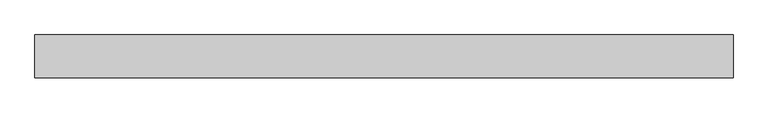
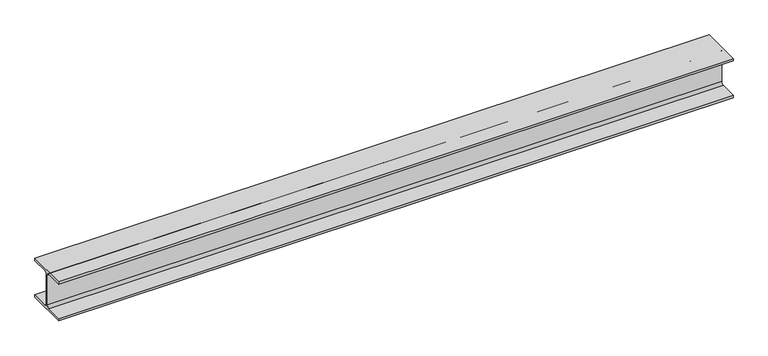
"""IFC4 building model written with IfcOpenShell, lengths in millimetres: beam geometry, 0912_Steel Framing_H-KSD3502 : H_SB_ASB_H-200x200x8x12."""

from ifc_helpers import new_model, si_unit, point, frame, frame_2d, origin, place, context, project, spatial, polyline, circle_curve, trimmed, segment, composite_curve, outline, extrude, source, transform, mapped, element, save


def beam_1c4525a5(model_context):
    return source(origin(), model_context, "Body", "SweptSolid", [
        extrude(outline(composite_curve([segment(polyline([(100.0, -88.0), (100.0, -100.0), (-100.0, -100.0), (-100.0, -88.0), (-17.0, -88.0)]), True, "CONTINUOUS"), segment(trimmed(circle_curve(frame_2d((-17.0, -75.0)), 13.0), [point((-17.0, -88.0))], [point((-4.0, -75.0))], True, "CARTESIAN"), True, "CONTINUOUS"), segment(polyline([(-4.0, -75.0), (-4.0, 75.0)]), True, "CONTINUOUS"), segment(trimmed(circle_curve(frame_2d((-17.0, 75.0)), 13.0), [point((-4.0, 75.0))], [point((-17.0, 88.0))], True, "CARTESIAN"), True, "CONTINUOUS"), segment(polyline([(-17.0, 88.0), (-100.0, 88.0), (-100.0, 100.0), (100.0, 100.0), (100.0, 88.0), (17.0, 88.0)]), True, "CONTINUOUS"), segment(trimmed(circle_curve(frame_2d((17.0, 75.0)), 13.0), [point((17.0, 88.0))], [point((4.0, 75.0))], True, "CARTESIAN"), True, "CONTINUOUS"), segment(polyline([(4.0, 75.0), (4.0, -75.0)]), True, "CONTINUOUS"), segment(trimmed(circle_curve(frame_2d((17.0, -75.0)), 13.0), [point((4.0, -75.0))], [point((17.0, -88.0))], True, "CARTESIAN"), True, "CONTINUOUS"), segment(polyline([(17.0, -88.0), (100.0, -88.0)]), True, "CONTINUOUS")], self_intersect=False)), frame((-1442.1256096, 0.0, 0.0), z_axis=(1.0, 0.0, 0.0), x_axis=(0.0, 1.0, 0.0)), (0.0, 0.0, 1.0), 3269.582171),
    ])


if __name__ == "__main__":
    model = new_model("IFC4")
    model_context = context("Model", 3, world=origin())
    ifc_project = project(units=[si_unit("LENGTHUNIT", "METRE", prefix="MILLI")], contexts=[model_context])
    site = spatial("IfcSite", under=ifc_project)
    building = spatial("IfcBuilding", under=site)
    placement = place(None, origin())
    beam_shape = beam_1c4525a5(model_context)
    element("IfcBeam", 1, ObjectType="0912_Steel Framing_H-KSD3502 : H_SB_ASB_H-200x200x8x12", at=placement, inside=building, context=model_context, shape_type="MappedRepresentation", body=[
        mapped(beam_shape, transform((0.0, 0.0, 0.0), x_axis=(1.0, 0.0, 0.0), y_axis=(0.0, 1.0, 0.0), z_axis=(0.0, 0.0, 1.0))),
    ])
    save(model, "model.ifc")

# Revit data of these elements
# Type "0912_Steel Framing_H-KSD3502 : H_SB_ASB_H-200x200x8x12"
#   H_WM Code_1 = "S01AA002-00001 | Main Steel Structure Fabrication Work | Shelter/Building | Medium Steel - Standard (90KG/M>Weight≥30KG/M) | Material: (   )"
#   H_WM Code_2 = "S03AA028-00001 | Main Steel Structure Erection Work | Shelter/Building | Medium Steel (90KG/M>Weight≥30KG/M) | Material: (   )"
#   H_WM Code_3 = "S01AA010-00001 | Main Steel Structure Fabrication Work | Shelter/Building | Steel Painting/Coating | for Non-Fireproofed Steel Surface, Surface Preparation, Primer, Second & Final Coat | Material: (   )"
#   H_Q'ty Cal Type Tag = "SB-Q2"
#   Width = 20.0 cm
#   Web Thickness = 0.8 cm
#   Web Fillet = 1.3 cm
#   Warping Constant = 141000.0 cm⁶
#   W = 0
#   Torsional Moment of Inertia = 26.2485 cm⁴
#   Section Area = 63.53 cm²
#   Plastic Modulus weak axis = 244.0 cm³
#   Plastic Modulus strong axis = 525.0 cm³
#   Perimeter = 1.16 m²/m
#   Nominal Weight = 49.90 kgf/m
#   Moment of Inertia weak axis = 1600.00 cm⁴
#   Moment of Inertia strong axis = 4720.00 cm⁴
#   Height = 20.0 cm
#   Flange Thickness = 1.2 cm
#   Elastic Modulus weak axis = 160.0 cm³
#   Elastic Modulus strong axis = 472.0 cm³
#   Centroid Vertical = 10.0 cm
#   Centroid Horizontal = 10.0 cm
#   Ix = 47200000
#   Length [instance default] = 1.5240 m
#   Zx = 525000
#   b = 0.2000 m
#   h = 0.2000 m
#   r = 0.0130 m
#   s = 0.0080 m
#   t = 0.0120 m
#   A = 0.006353 m²
#   Structural Material [instance default] = Steel, 45-345
#   Assembly Code = ""
# Element 1 (IfcBeam, "0912_Steel Framing_H-KSD3502 : H_SB_ASB_H-200x200x8x12")
#   Structural Material = none
# Materials
#   "Steel, 45-345": class "Metal", colour RGB 189 187 185, transparency 0, Description = "Steel 345 MPa", Cost = 0
